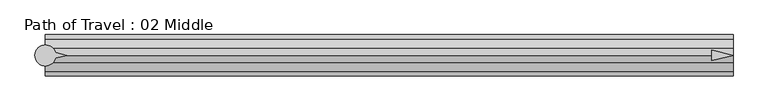
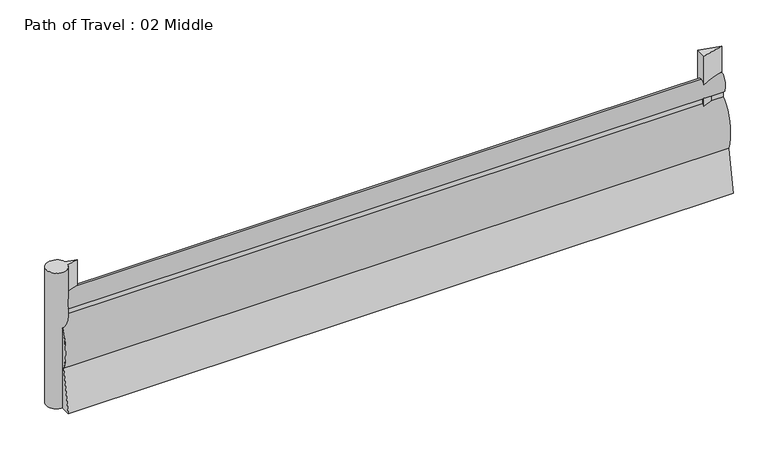
"""IFC4 building model written with IfcOpenShell, lengths in millimetres: proxy geometry, Path of Travel : 02 Middle."""

from ifc_helpers import new_model, si_unit, point, frame, frame_2d, origin, origin_with_axes, place, context, project, spatial, polyline, circle_curve, ellipse_curve, trimmed, segment, composite_curve, outline, extrude, source, transform, mapped, element, save
from ifc_brep_helpers import plane_surface, extruded_surface, advanced_brep


def path_of_travel_02_middle_bddeb292(model_context):
    return source(origin(), model_context, "Body", "SolidModel", [
        advanced_brep(
        [(227.5554837, 0.0, 1727.2), (227.5554837, 42.9018657, 1436.6534209), (227.5554837, 42.9018657, 1363.4763406), (227.5554837, 184.1186263, 643.4144547), (227.5554837, 297.5699544, 0.0), (227.5554837, 145.6574193, 0.0), (227.5554837, 0.0, 584.2), (227.5554837, -145.6574193, 0.0), (227.5554837, -297.5699544, 0.0), (227.5554837, -184.1186263, 643.4144547), (227.5554837, -42.9018657, 1363.4763406), (227.5554837, -42.9018657, 1436.6534209), (10109.432065, 0.0, 1727.2), (10109.432065, -42.9018657, 1436.6534209), (10109.432065, -42.9018657, 1363.4763406), (10109.432065, -184.1186263, 643.4144547), (10109.432065, -297.5699544, 0.0), (10109.432065, -145.6574193, 0.0), (10109.432065, 0.0, 584.2), (10109.432065, 145.6574193, 0.0), (10109.432065, 297.5699544, 0.0), (10109.432065, 184.1186263, 643.4144547), (10109.432065, 42.9018657, 1363.4763406), (10109.432065, 42.9018657, 1436.6534209)],
        [
            (0, 1, ellipse_curve(frame((227.5554837, 0.0, 1574.8), z_axis=(-1.0, 0.0, 0.0), x_axis=(0.0, 0.0, 1.0)), 152.4, 101.6)),
            (1, 2),
            (2, 3, ellipse_curve(frame((227.5554837, 0.0, 914.4), z_axis=(-1.0, 0.0, 0.0), x_axis=(0.0, 0.0, -1.0)), 457.2, 228.6)),
            (3, 4),
            (4, 5),
            (5, 6),
            (6, 7),
            (7, 8),
            (8, 9),
            (9, 10, ellipse_curve(frame((227.5554837, 0.0, 914.4), z_axis=(-1.0, 0.0, 0.0), x_axis=(0.0, 0.0, -1.0)), 457.2, 228.6)),
            (10, 11),
            (11, 0, ellipse_curve(frame((227.5554837, 0.0, 1574.8), z_axis=(-1.0, 0.0, 0.0), x_axis=(0.0, 0.0, 1.0)), 152.4, 101.6)),
            (12, 13, ellipse_curve(frame((10109.432065, 0.0, 1574.8), z_axis=(1.0, 0.0, 0.0), x_axis=(0.0, 0.0, 1.0)), 152.4, 101.6)),
            (13, 14),
            (14, 15, ellipse_curve(frame((10109.432065, 0.0, 914.4), z_axis=(1.0, 0.0, 0.0), x_axis=(0.0, 0.0, -1.0)), 457.2, 228.6)),
            (15, 16),
            (16, 17),
            (17, 18),
            (18, 19),
            (19, 20),
            (20, 21),
            (21, 22, ellipse_curve(frame((10109.432065, 0.0, 914.4), z_axis=(1.0, 0.0, 0.0), x_axis=(0.0, 0.0, -1.0)), 457.2, 228.6)),
            (22, 23),
            (23, 12, ellipse_curve(frame((10109.432065, 0.0, 1574.8), z_axis=(1.0, 0.0, 0.0), x_axis=(0.0, 0.0, 1.0)), 152.4, 101.6)),
            (0, 12),
            (23, 1),
            (22, 2),
            (21, 3),
            (20, 4),
            (19, 5),
            (18, 6),
            (17, 7),
            (16, 8),
            (15, 9),
            (14, 10),
            (13, 11),
        ],
        [
            plane_surface(frame((227.5554837, 0.0, 0.0), z_axis=(-1.0, 0.0, 0.0), x_axis=(0.0, 0.0, 1.0))),
            plane_surface(frame((10109.432065, 0.0, 0.0), z_axis=(1.0, 0.0, 0.0), x_axis=(0.0, 0.0, 1.0))),
            extruded_surface(trimmed(ellipse_curve(frame((10109.432065, 0.0, 1574.8), z_axis=(-1.0, 0.0, 0.0), x_axis=(0.0, 0.0, 1.0)), 152.4, 101.6), [point((10109.432065, 0.0, 1727.2))], [point((10109.432065, 42.9018657, 1436.6534209))], True, "CARTESIAN"), (-9881.8765813, 0.0, 0.0), 9881.8765813),
            plane_surface(frame((227.5554837, 42.9018657, 1436.6534209), z_axis=(0.0, 1.0, 0.0), x_axis=(1.0, 0.0, 0.0))),
            extruded_surface(trimmed(ellipse_curve(frame((10109.432065, 0.0, 914.4), z_axis=(-1.0, 0.0, 0.0), x_axis=(0.0, 0.0, -1.0)), 457.2, 228.6), [point((10109.432065, 42.9018657, 1363.4763406))], [point((10109.432065, 184.1186263, 643.4144547))], True, "CARTESIAN"), (-9881.8765813, 0.0, 0.0), 9881.8765813),
            plane_surface(frame((227.5554837, 184.1186263, 643.4144547), z_axis=(0.0, 0.9848077530122078, 0.1736481776669322), x_axis=(1.0, 0.0, 0.0))),
            plane_surface(frame((227.5554837, 297.5699544, 0.0), z_axis=(0.0, 0.0, -1.0), x_axis=(1.0, 0.0, 0.0))),
            plane_surface(frame((227.5554837, 145.6574193, 0.0), z_axis=(0.0, -0.9702957262760199, -0.2419218955995739), x_axis=(1.0, 0.0, 0.0))),
            plane_surface(frame((227.5554837, 0.0, 584.2), z_axis=(0.0, 0.9702957262759961, -0.24192189559966923), x_axis=(1.0, 0.0, 0.0))),
            plane_surface(frame((227.5554837, -145.6574193, 0.0), z_axis=(0.0, 0.0, -1.0), x_axis=(1.0, 0.0, 0.0))),
            plane_surface(frame((227.5554837, -297.5699544, 0.0), z_axis=(0.0, -0.984807753012208, 0.17364817766693066), x_axis=(1.0, 0.0, 0.0))),
            extruded_surface(trimmed(ellipse_curve(frame((10109.432065, 0.0, 914.4), z_axis=(-1.0, 0.0, 0.0), x_axis=(0.0, 0.0, -1.0)), 457.2, 228.6), [point((10109.432065, -184.1186263, 643.4144547))], [point((10109.432065, -42.9018657, 1363.4763406))], True, "CARTESIAN"), (-9881.8765813, 0.0, 0.0), 9881.8765813),
            plane_surface(frame((227.5554837, -42.9018657, 1363.4763406), z_axis=(0.0, -1.0, 0.0), x_axis=(1.0, 0.0, 0.0))),
            extruded_surface(trimmed(ellipse_curve(frame((10109.432065, 0.0, 1574.8), z_axis=(-1.0, 0.0, 0.0), x_axis=(0.0, 0.0, 1.0)), 152.4, 101.6), [point((10109.432065, -42.9018657, 1436.6534209))], [point((10109.432065, 0.0, 1727.2))], True, "CARTESIAN"), (-9881.8765813, 0.0, 0.0), 9881.8765813),
        ],
        [
            (0, [[1, 2, 3, 4, 5, 6, 7, 8, 9, 10, 11, 12]]),
            (1, [[13, 14, 15, 16, 17, 18, 19, 20, 21, 22, 23, 24]]),
            (2, [[-1, 25, -24, 26]]),
            (3, [[-2, -26, -23, 27]]),
            (4, [[-3, -27, -22, 28]]),
            (5, [[-4, -28, -21, 29]]),
            (6, [[-5, -29, -20, 30]]),
            (7, [[-6, -30, -19, 31]]),
            (8, [[-7, -31, -18, 32]]),
            (9, [[-8, -32, -17, 33]]),
            (10, [[-9, -33, -16, 34]]),
            (11, [[-10, -34, -15, 35]]),
            (12, [[-11, -35, -14, 36]]),
            (13, [[-12, -36, -13, -25]]),
        ],
    ),
        extrude(outline(polyline([(9803.4269185, 76.2006338), (10109.432065, 0.0), (9803.4269185, -76.2006338), (9803.4269185, 76.2006338)])), origin_with_axes(), (0.0, 0.0, 1.0), 2129.5973753),
        extrude(outline(composite_curve([segment(polyline([(372.7837828, 39.4440225), (531.182385, 0.0), (372.7837828, -39.4440225)]), True, "CONTINUOUS"), segment(trimmed(circle_curve(frame_2d((227.2200886, 0.0)), 150.8131956), [point((372.7837828, -39.4440225))], [point((372.7837828, 39.4440225))], False, "CARTESIAN"), True, "CONTINUOUS")], self_intersect=False)), origin_with_axes(), (0.0, 0.0, 1.0), 2129.5973753),
    ])


if __name__ == "__main__":
    model = new_model("IFC4")
    model_context = context("Model", 3, world=origin())
    ifc_project = project(units=[si_unit("LENGTHUNIT", "METRE", prefix="MILLI")], contexts=[model_context])
    site = spatial("IfcSite", under=ifc_project)
    building = spatial("IfcBuilding", under=site)
    placement = place(None, origin())
    path_of_travel_02_middle_shape = path_of_travel_02_middle_bddeb292(model_context)
    element("IfcBuildingElementProxy", 1, Name="Path of Travel : 02 Middle", ObjectType="Path of Travel : 02 Middle", at=placement, inside=building, context=model_context, shape_type="MappedRepresentation", body=[
        mapped(path_of_travel_02_middle_shape, transform((0.0, 0.0, 0.0), x_axis=(1.0, 0.0, 0.0), y_axis=(0.0, 1.0, 0.0), z_axis=(0.0, 0.0, 1.0))),
    ])
    save(model, "model.ifc")

# Revit data of these elements
# Type "Path of Travel : 02 Middle"
#   Path of Egress [instance default] = 4' - 0"
#   built-in parameter 1001306 [instance default] = 4 (stored number, unit not read)
#   Dot at Start = no
#   Arrow in Middle = yes
#   Arrow at End = no
#   Egress Path = none
# Element 1 (IfcBuildingElementProxy, "Path of Travel : 02 Middle")
#   Path of Egress = 32' - 5.05026"
#   built-in parameter 1001306 = 32.4209 (stored number, unit not read)
